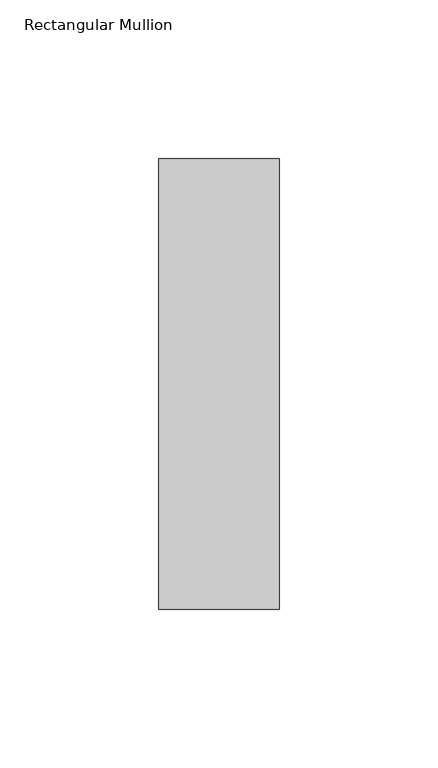
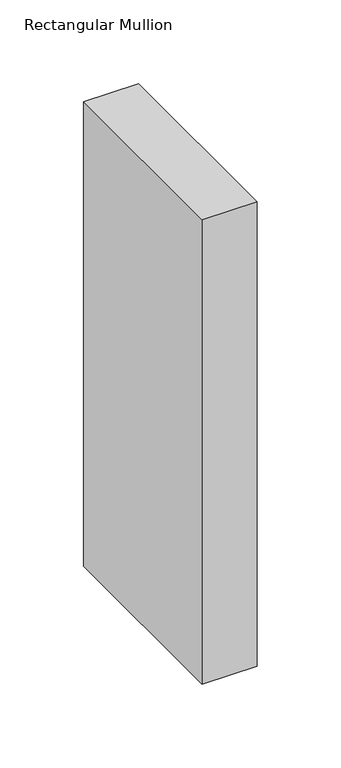
"""IFC4 building model written with IfcOpenShell, lengths in millimetres: member geometry, Rectangular Mullion : NLRS_21_CWM_hsb-regel 38x142_gen_rsf."""

from ifc_helpers import new_model, si_unit, frame, origin, place, context, project, spatial, polyline, outline, extrude, source, transform, mapped, element, save


def rectangular_mullion_1e8108f6(model_context):
    return source(origin(), model_context, "Body", "SweptSolid", [
        extrude(outline(polyline([(19.0, -71.0), (-19.0, -71.0), (-19.0, 71.0), (19.0, 71.0), (19.0, -71.0)])), frame((0.0, 0.0, -339.0041412), z_axis=(0.0, 0.0, 1.0), x_axis=(1.0, 0.0, 0.0)), (0.0, 0.0, 1.0), 339.0041412),
    ])


if __name__ == "__main__":
    model = new_model("IFC4")
    model_context = context("Model", 3, world=origin())
    ifc_project = project(units=[si_unit("LENGTHUNIT", "METRE", prefix="MILLI")], contexts=[model_context])
    site = spatial("IfcSite", under=ifc_project)
    building = spatial("IfcBuilding", under=site)
    placement = place(None, origin())
    rectangular_mullion_shape = rectangular_mullion_1e8108f6(model_context)
    element("IfcMember", 1, ObjectType="Rectangular Mullion : NLRS_21_CWM_hsb-regel 38x142_gen_rsf", at=placement, inside=building, context=model_context, shape_type="MappedRepresentation", body=[
        mapped(rectangular_mullion_shape, transform((0.0, 0.0, 0.0), x_axis=(1.0, 0.0, 0.0), y_axis=(0.0, 1.0, 0.0), z_axis=(0.0, 0.0, 1.0))),
    ])
    save(model, "model.ifc")

# Revit data of these elements
# Type "Rectangular Mullion : NLRS_21_CWM_hsb-regel 38x142_gen_rsf"
#   Export Type to IFC As = "IfcWall"
#   Type IfcGUID = "07M7mRoiH1CR8m_RSKIwpF"
#   Assembly Code = "21.10"
#   built-in parameter 1007322 = 0.465879 (stored number, unit not read)
#   built-in parameter 1007321 = 0.062336 (stored number, unit not read)
#   built-in parameter 1007320 = 0.062336 (stored number, unit not read)
# Element 1 (IfcMember, "Rectangular Mullion : NLRS_21_CWM_hsb-regel 38x142_gen_rsf")
#   Materials on its faces: "NLRS_i2_hout naaldhout vuren_gen_rsf"
# Materials
#   "NLRS_i2_hout naaldhout vuren_gen_rsf": class "I - Hout", colour RGB 234 199 147, transparency 0, Keynote = "i2", Manufacturer = "Revit Standards Foundation", URL = "www.revitstandards.org", Description = "hout vuren", Cost = 0
